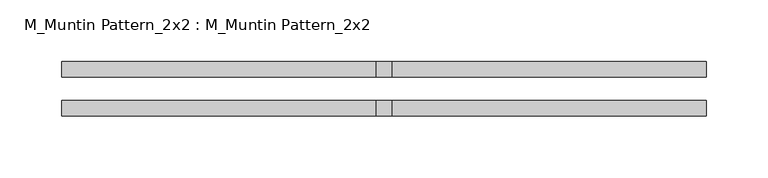
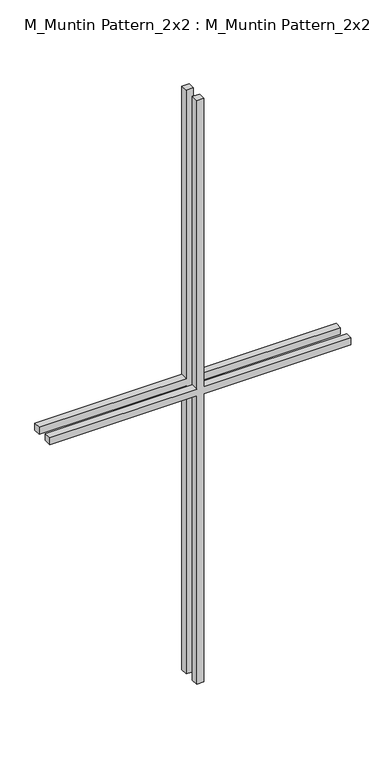
"""IFC4 building model written with IfcOpenShell, lengths in millimetres: proxy geometry, M_Muntin Pattern_2x2 : M_Muntin Pattern_2x2."""

from ifc_helpers import new_model, si_unit, frame, origin, place, context, project, spatial, polyline, outline, extrude, source, transform, mapped, element, save


def m_muntin_pattern_2x2_m_muntin_pattern_2x2_cf37b409(model_context):
    return source(origin(), model_context, "Body", "SweptSolid", [
        extrude(outline(polyline([(542.925, -6.35), (542.925, -261.9375), (530.225, -261.9375), (530.225, -6.35), (0.0, -6.35), (0.0, 6.35), (530.225, 6.35), (530.225, 261.9375), (542.925, 261.9375), (542.925, 6.35), (1073.15, 6.35), (1073.15, -6.35), (542.925, -6.35)])), frame((0.0, 9.525, 0.0), z_axis=(0.0, 1.0, 0.0), x_axis=(0.0, 0.0, 1.0)), (0.0, 0.0, 1.0), 12.7),
        extrude(outline(polyline([(542.925, -6.35), (542.925, -261.9375), (530.225, -261.9375), (530.225, -6.35), (0.0, -6.35), (0.0, 6.35), (530.225, 6.35), (530.225, 261.9375), (542.925, 261.9375), (542.925, 6.35), (1073.15, 6.35), (1073.15, -6.35), (542.925, -6.35)])), frame((0.0, -22.225, 0.0), z_axis=(0.0, 1.0, 0.0), x_axis=(0.0, 0.0, 1.0)), (0.0, 0.0, 1.0), 12.7),
    ])


if __name__ == "__main__":
    model = new_model("IFC4")
    model_context = context("Model", 3, world=origin())
    ifc_project = project(units=[si_unit("LENGTHUNIT", "METRE", prefix="MILLI")], contexts=[model_context])
    site = spatial("IfcSite", under=ifc_project)
    building = spatial("IfcBuilding", under=site)
    placement = place(None, origin())
    m_muntin_pattern_2x2_m_muntin_pattern_2x2_shape = m_muntin_pattern_2x2_m_muntin_pattern_2x2_cf37b409(model_context)
    element("IfcBuildingElementProxy", 1, Name="M_Muntin Pattern_2x2 : M_Muntin Pattern_2x2", ObjectType="M_Muntin Pattern_2x2 : M_Muntin Pattern_2x2", at=placement, inside=building, context=model_context, shape_type="MappedRepresentation", body=[
        mapped(m_muntin_pattern_2x2_m_muntin_pattern_2x2_shape, transform((0.0, 0.0, 0.0), x_axis=(1.0, 0.0, 0.0), y_axis=(0.0, 1.0, 0.0), z_axis=(0.0, 0.0, 1.0))),
    ])
    save(model, "model.ifc")

# Revit data of these elements
# Type "M_Muntin Pattern_2x2 : M_Muntin Pattern_2x2"
#   Width [instance default] = 3' - 11.24409"
#   Thickness = 0' - 0 1/2"
#   Height [instance default] = 3' - 11.24409"
#   Distance = 0' - 0 3/4"
#   Interior Material [instance default] = none
#   Exterior Material [instance default] = none
#   Default Elevation = 0
# Element 1 (IfcBuildingElementProxy, "M_Muntin Pattern_2x2 : M_Muntin Pattern_2x2")
#   Width = 1' - 8 5/8"
#   Height = 3' - 6 1/4"
#   Interior Material = Wood - Stained
#   Exterior Material = Clad - White
#   Materials on its faces: "Clad - White", "Wood - Stained"
# Materials
#   "Clad - White": class "Wood", colour RGB 242 242 238, transparency 0, Cost = 0
#   "Wood - Stained": class "Wood", colour RGB 224 178 126, transparency 0, Cost = 0
